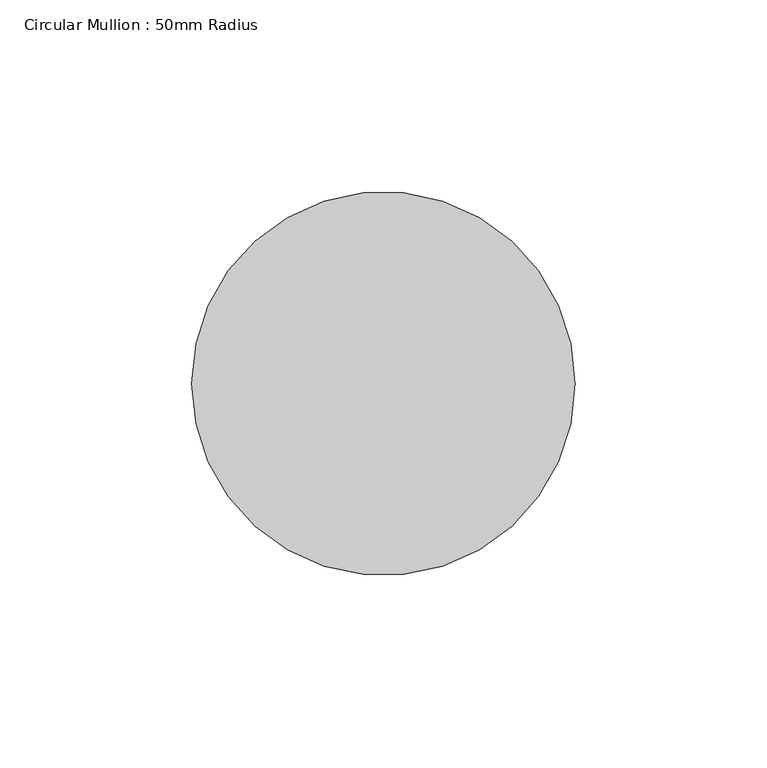
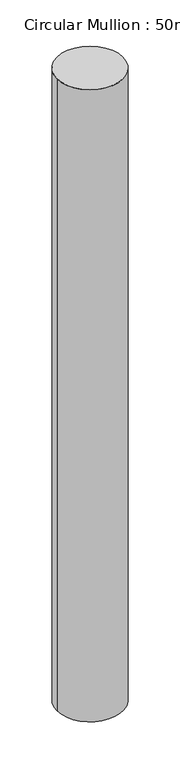
"""IFC4 building model written with IfcOpenShell, lengths in millimetres: member geometry, Circular Mullion : 50mm Radius."""

from ifc_helpers import new_model, si_unit, point, frame, origin, origin_2d, place, context, project, spatial, circle_curve, trimmed, segment, composite_curve, outline, extrude, source, transform, mapped, element, save


def circular_mullion_50mm_radius_a0008a5c(model_context):
    return source(origin(), model_context, "Body", "SweptSolid", [
        extrude(outline(composite_curve([segment(trimmed(circle_curve(origin_2d(), 50.0), [point((50.0, 0.0))], [point((-50.0, 0.0))], False, "CARTESIAN"), True, "CONTINUOUS"), segment(trimmed(circle_curve(origin_2d(), 50.0), [point((-50.0, 0.0))], [point((50.0, 0.0))], False, "CARTESIAN"), True, "CONTINUOUS")], self_intersect=False)), frame((0.0, 0.0, -1011.6543074), z_axis=(0.0, 0.0, 1.0), x_axis=(1.0, 0.0, 0.0)), (0.0, 0.0, 1.0), 1011.6543074),
    ])


if __name__ == "__main__":
    model = new_model("IFC4")
    model_context = context("Model", 3, world=origin())
    ifc_project = project(units=[si_unit("LENGTHUNIT", "METRE", prefix="MILLI")], contexts=[model_context])
    site = spatial("IfcSite", under=ifc_project)
    building = spatial("IfcBuilding", under=site)
    placement = place(None, origin())
    circular_mullion_50mm_radius_shape = circular_mullion_50mm_radius_a0008a5c(model_context)
    element("IfcMember", 1, ObjectType="Circular Mullion : 50mm Radius", at=placement, inside=building, context=model_context, shape_type="MappedRepresentation", body=[
        mapped(circular_mullion_50mm_radius_shape, transform((0.0, 0.0, 0.0), x_axis=(1.0, 0.0, 0.0), y_axis=(0.0, 1.0, 0.0), z_axis=(0.0, 0.0, 1.0))),
    ])
    save(model, "model.ifc")

# Revit data of these elements
# Type "Circular Mullion : 50mm Radius"
#   built-in parameter 1007350 = 0.164042 (stored number, unit not read)
# Element 1 (IfcMember, "Circular Mullion : 50mm Radius")
#   Materials on its faces: "Aluminium"
# Materials
#   "Aluminium": class "Metal", colour RGB 247 247 247, transparency 0, Description = "Aluminium 6061", Cost = 0
